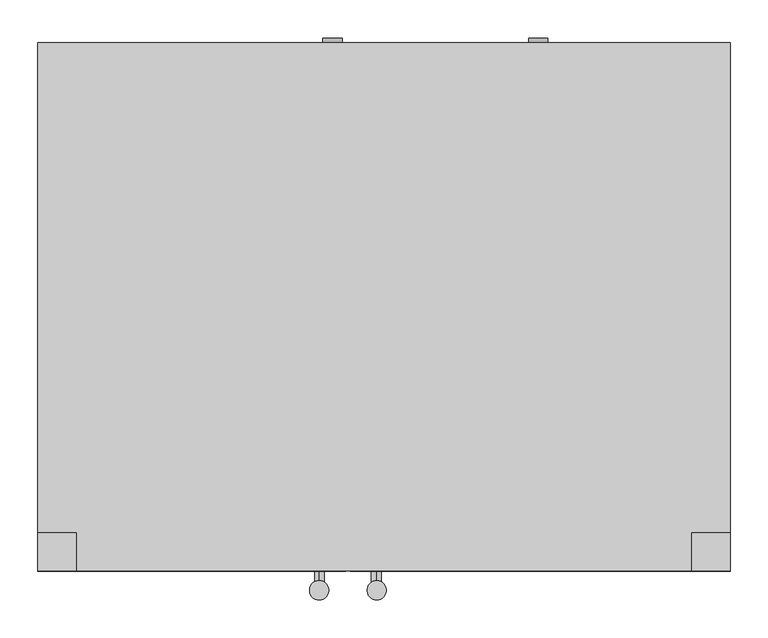
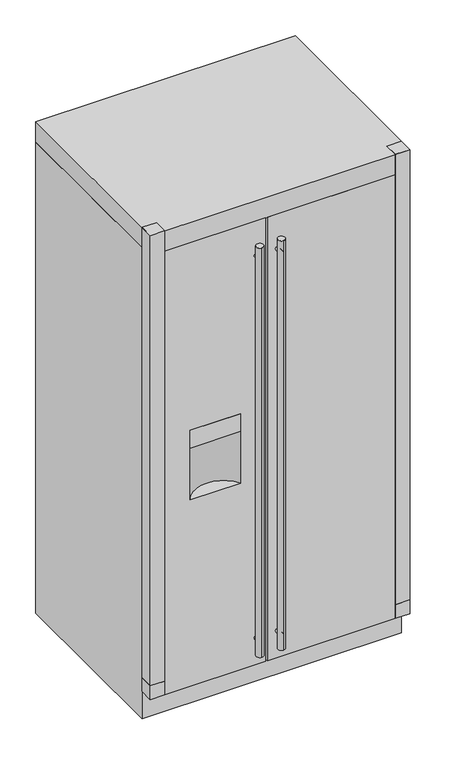
"""IFC4 building model written with IfcOpenShell, lengths in millimetres: proxy geometry, Refrige_Side-By-Side_GE-Monogram_ZFSB23DXSS : Refrige_Side-By-Side_GE-Monogram_ZFSB23DXSS."""

from ifc_helpers import new_model, si_unit, point, frame, frame_2d, origin, origin_with_axes, place, context, project, spatial, polyline, circle_curve, trimmed, segment, composite_curve, outline, extrude, faceted_brep, source, transform, mapped, element, save
from ifc_brep_helpers import plane_surface, revolved_surface, advanced_brep


def specialty_equipment_95538555(model_context):
    return source(origin(), model_context, "Body", "SolidModel", [
        extrude(outline(composite_curve([segment(trimmed(circle_curve(frame_2d((203.2, -10.2065026)), 6.35), [point((196.85, -10.2065026))], [point((209.55, -10.2065026))], False, "CARTESIAN"), True, "CONTINUOUS"), segment(trimmed(circle_curve(frame_2d((203.2, -10.2065026)), 6.35), [point((209.55, -10.2065026))], [point((196.85, -10.2065026))], False, "CARTESIAN"), True, "CONTINUOUS")], self_intersect=False)), frame((0.0, -546.1, 0.0), z_axis=(0.0, 1.0, 0.0), x_axis=(0.0, 0.0, 1.0)), (0.0, 0.0, 1.0), 25.4),
        extrude(outline(composite_curve([segment(trimmed(circle_curve(frame_2d((1625.6, -10.2065026)), 6.35), [point((1619.25, -10.2065026))], [point((1631.95, -10.2065026))], False, "CARTESIAN"), True, "CONTINUOUS"), segment(trimmed(circle_curve(frame_2d((1625.6, -10.2065026)), 6.35), [point((1631.95, -10.2065026))], [point((1619.25, -10.2065026))], False, "CARTESIAN"), True, "CONTINUOUS")], self_intersect=False)), frame((0.0, -546.1, 0.0), z_axis=(0.0, 1.0, 0.0), x_axis=(0.0, 0.0, 1.0)), (0.0, 0.0, 1.0), 25.4),
        extrude(outline(composite_curve([segment(trimmed(circle_curve(frame_2d((-9.7026178, -546.1)), 12.7), [point((-9.7026178, -558.8))], [point((-9.7026178, -533.4))], False, "CARTESIAN"), True, "CONTINUOUS"), segment(trimmed(circle_curve(frame_2d((-9.7026178, -546.1)), 12.7), [point((-9.7026178, -533.4))], [point((-9.7026178, -558.8))], False, "CARTESIAN"), True, "CONTINUOUS")], self_intersect=False)), frame((0.0, 0.0, 152.4), z_axis=(0.0, 0.0, 1.0), x_axis=(1.0, 0.0, 0.0)), (0.0, 0.0, 1.0), 1524.0),
        extrude(outline(composite_curve([segment(trimmed(circle_curve(frame_2d((203.2, -85.1990605)), 6.35), [point((196.85, -85.1990605))], [point((209.55, -85.1990605))], False, "CARTESIAN"), True, "CONTINUOUS"), segment(trimmed(circle_curve(frame_2d((203.2, -85.1990605)), 6.35), [point((209.55, -85.1990605))], [point((196.85, -85.1990605))], False, "CARTESIAN"), True, "CONTINUOUS")], self_intersect=False)), frame((0.0, -546.1, 0.0), z_axis=(0.0, 1.0, 0.0), x_axis=(0.0, 0.0, 1.0)), (0.0, 0.0, 1.0), 25.4),
        extrude(outline(composite_curve([segment(trimmed(circle_curve(frame_2d((1625.6, -85.1990605)), 6.35), [point((1619.25, -85.1990605))], [point((1631.95, -85.1990605))], False, "CARTESIAN"), True, "CONTINUOUS"), segment(trimmed(circle_curve(frame_2d((1625.6, -85.1990605)), 6.35), [point((1631.95, -85.1990605))], [point((1619.25, -85.1990605))], False, "CARTESIAN"), True, "CONTINUOUS")], self_intersect=False)), frame((0.0, -546.1, 0.0), z_axis=(0.0, 1.0, 0.0), x_axis=(0.0, 0.0, 1.0)), (0.0, 0.0, 1.0), 25.4),
        extrude(outline(composite_curve([segment(trimmed(circle_curve(frame_2d((-85.7029453, -546.1)), 12.7), [point((-85.7029453, -558.8))], [point((-85.7029453, -533.4))], False, "CARTESIAN"), True, "CONTINUOUS"), segment(trimmed(circle_curve(frame_2d((-85.7029453, -546.1)), 12.7), [point((-85.7029453, -533.4))], [point((-85.7029453, -558.8))], False, "CARTESIAN"), True, "CONTINUOUS")], self_intersect=False)), frame((0.0, 0.0, 152.4), z_axis=(0.0, 0.0, 1.0), x_axis=(1.0, 0.0, 0.0)), (0.0, 0.0, 1.0), 1524.0),
        extrude(outline(composite_curve([segment(trimmed(circle_curve(frame_2d((-228.6, -573.0875)), 103.1875), [point((-317.5, -520.7))], [point((-139.7, -520.7))], False, "CARTESIAN"), True, "CONTINUOUS"), segment(polyline([(-139.7, -520.7), (-317.5, -520.7)]), True, "CONTINUOUS")], self_intersect=False)), frame((0.0, 0.0, 989.0466464), z_axis=(0.0, 0.0, 1.0), x_axis=(1.0, 0.0, 0.0)), (0.0, 0.0, 1.0), 65.7299795),
        extrude(outline(polyline([(-406.4, -469.9), (-406.4, -520.7), (-457.2, -520.7), (-457.2, -469.9), (-406.4, -469.9)])), frame((0.0, 0.0, 101.6), z_axis=(0.0, 0.0, 1.0), x_axis=(1.0, 0.0, 0.0)), (0.0, 0.0, 1.0), 50.8),
        extrude(outline(polyline([(457.2, -469.9), (457.2, -520.7), (406.4, -520.7), (406.4, -469.9), (457.2, -469.9)])), frame((0.0, 0.0, 101.6), z_axis=(0.0, 0.0, 1.0), x_axis=(1.0, 0.0, 0.0)), (0.0, 0.0, 1.0), 50.8),
        extrude(outline(polyline([(-406.4, -469.9), (-406.4, -520.7), (-457.2, -520.7), (-457.2, -469.9), (-406.4, -469.9)])), frame((0.0, 0.0, 101.6), z_axis=(0.0, 0.0, 1.0), x_axis=(1.0, 0.0, 0.0)), (0.0, 0.0, 1.0), 1727.2),
        extrude(outline(polyline([(406.4, -469.9), (457.2, -469.9), (457.2, -520.7), (406.4, -520.7), (406.4, -469.9)])), frame((0.0, 0.0, 101.6), z_axis=(0.0, 0.0, 1.0), x_axis=(1.0, 0.0, 0.0)), (0.0, 0.0, 1.0), 1727.2),
        advanced_brep(
        [(-50.8, -469.9, 1752.6), (-406.4, -469.9, 1752.6), (-406.4, -520.7, 1752.6), (-50.8, -520.7, 1752.6), (-50.8, -469.9, 101.6), (-50.8, -520.7, 101.6), (-406.4, -520.7, 101.6), (-406.4, -469.9, 101.6), (-317.5, -520.7, 1054.7766259), (-139.7, -520.7, 1054.7766259), (-139.7, -520.7, 796.7567269), (-317.5, -520.7, 796.7567269), (-228.6, -469.9, 1054.7766259), (-228.6, -469.9, 796.7567269)],
        [
            (0, 1),
            (1, 2),
            (2, 3),
            (3, 0),
            (4, 5),
            (5, 6),
            (6, 7),
            (7, 4),
            (0, 4),
            (7, 1),
            (6, 2),
            (5, 3),
            (8, 9),
            (9, 10),
            (10, 11),
            (11, 8),
            (8, 12, circle_curve(frame((-228.6, -573.0875, 1054.7766259), z_axis=(0.0, 0.0, -1.0), x_axis=(1.0, 0.0, 0.0)), 103.1875)),
            (12, 9, circle_curve(frame((-228.6, -573.0875, 1054.7766259), z_axis=(0.0, 0.0, -1.0), x_axis=(1.0, 0.0, 0.0)), 103.1875)),
            (10, 13, circle_curve(frame((-228.6, -573.0875, 796.7567269), z_axis=(0.0, 0.0, 1.0), x_axis=(1.0, 0.0, 0.0)), 103.1875)),
            (13, 11, circle_curve(frame((-228.6, -573.0875, 796.7567269), z_axis=(0.0, 0.0, 1.0), x_axis=(1.0, 0.0, 0.0)), 103.1875)),
        ],
        [
            plane_surface(frame((-406.4, -469.9, 1752.6), z_axis=(0.0, 0.0, 1.0), x_axis=(-1.0, 0.0, 0.0))),
            plane_surface(frame((-406.4, -469.9, 101.6), z_axis=(0.0, 0.0, -1.0), x_axis=(1.0, 0.0, 0.0))),
            plane_surface(frame((-50.8, -469.9, 1752.6), z_axis=(0.0, 1.0, 0.0), x_axis=(0.0, 0.0, -1.0))),
            plane_surface(frame((-406.4, -469.9, 1752.6), z_axis=(-1.0, 0.0, 0.0), x_axis=(0.0, 0.0, -1.0))),
            plane_surface(frame((-406.4, -520.7, 1752.6), z_axis=(0.0, -1.0, 0.0), x_axis=(0.0, 0.0, -1.0))),
            plane_surface(frame((-50.8, -520.7, 1752.6), z_axis=(1.0, 0.0, 0.0), x_axis=(0.0, 0.0, -1.0))),
            plane_surface(frame((-139.7, -520.7, 1054.7766259), z_axis=(0.0, 0.0, -1.0), x_axis=(1.0, 0.0, 0.0))),
            plane_surface(frame((-139.7, -520.7, 796.7567269), z_axis=(0.0, 0.0, 1.0), x_axis=(-1.0, 0.0, 0.0))),
            revolved_surface(polyline([(-125.4125, -573.0875, 1054.7766259), (-125.4125, -573.0875, 796.7567269)]), (-228.6, -573.0875, 796.7567269), (0.0, 0.0, 1.0)),
        ],
        [
            (0, [[1, 2, 3, 4]]),
            (1, [[5, 6, 7, 8]]),
            (2, [[-1, 9, -8, 10]]),
            (3, [[-2, -10, -7, 11]]),
            (4, [[-3, -11, -6, 12], [13, 14, 15, 16]]),
            (5, [[-4, -12, -5, -9]]),
            (6, [[17, 18, -13]]),
            (7, [[19, 20, -15]]),
            (8, [[-17, -16, -20, -19, -14, -18]]),
        ],
    ),
        faceted_brep([(406.4, -469.9, 1752.6), (-44.45, -469.9, 1752.6), (-44.45, -520.7, 1752.6), (406.4, -520.7, 1752.6), (406.4, -469.9, 101.6), (406.4, -520.7, 101.6), (-44.45, -520.7, 101.6), (-44.45, -469.9, 101.6)], [[[0, 1, 2, 3]], [[4, 5, 6, 7]], [[1, 0, 4, 7]], [[2, 1, 7, 6]], [[3, 2, 6, 5]], [[0, 3, 5, 4]]]),
        extrude(outline(polyline([(457.2, -469.9), (-457.2, -469.9), (-457.2, 177.8), (457.2, 177.8), (457.2, -469.9)])), origin_with_axes(), (0.0, 0.0, 1.0), 1752.6),
        extrude(outline(polyline([(-457.2, -520.7), (-457.2, 177.8), (457.2, 177.8), (457.2, -520.7), (-457.2, -520.7)])), frame((0.0, 0.0, 1752.6), z_axis=(0.0, 0.0, 1.0), x_axis=(1.0, 0.0, 0.0)), (0.0, 0.0, 1.0), 76.2),
        extrude(outline(composite_curve([segment(trimmed(circle_curve(frame_2d((314.6288473, -68.0887314)), 12.7), [point((314.6288473, -55.3887314))], [point((314.6288473, -80.7887314))], False, "CARTESIAN"), True, "CONTINUOUS"), segment(trimmed(circle_curve(frame_2d((314.6288473, -68.0887314)), 12.7), [point((314.6288473, -80.7887314))], [point((314.6288473, -55.3887314))], False, "CARTESIAN"), True, "CONTINUOUS")], self_intersect=False)), frame((0.0, 177.8, 0.0), z_axis=(0.0, 1.0, 0.0), x_axis=(0.0, 0.0, 1.0)), (0.0, 0.0, 1.0), 6.35),
        extrude(outline(composite_curve([segment(trimmed(circle_curve(frame_2d((314.6288473, 203.7929589)), 12.7), [point((314.6288473, 216.4929589))], [point((314.6288473, 191.0929589))], False, "CARTESIAN"), True, "CONTINUOUS"), segment(trimmed(circle_curve(frame_2d((314.6288473, 203.7929589)), 12.7), [point((314.6288473, 191.0929589))], [point((314.6288473, 216.4929589))], False, "CARTESIAN"), True, "CONTINUOUS")], self_intersect=False)), frame((0.0, 177.8, 0.0), z_axis=(0.0, 1.0, 0.0), x_axis=(0.0, 0.0, 1.0)), (0.0, 0.0, 1.0), 6.35),
    ])


if __name__ == "__main__":
    model = new_model("IFC4")
    model_context = context("Model", 3, world=origin())
    ifc_project = project(units=[si_unit("LENGTHUNIT", "METRE", prefix="MILLI")], contexts=[model_context])
    site = spatial("IfcSite", under=ifc_project)
    building = spatial("IfcBuilding", under=site)
    placement = place(None, origin())
    specialty_equipment_shape = specialty_equipment_95538555(model_context)
    element("IfcBuildingElementProxy", 1, Name="Refrige_Side-By-Side_GE-Monogram_ZFSB23DXSS : Refrige_Side-By-Side_GE-Monogram_ZFSB23DXSS", ObjectType="Refrige_Side-By-Side_GE-Monogram_ZFSB23DXSS : Refrige_Side-By-Side_GE-Monogram_ZFSB23DXSS", at=placement, inside=building, context=model_context, shape_type="MappedRepresentation", body=[
        mapped(specialty_equipment_shape, transform((0.0, 0.0, 0.0), x_axis=(1.0, 0.0, 0.0), y_axis=(0.0, 1.0, 0.0), z_axis=(0.0, 0.0, 1.0))),
    ])
    save(model, "model.ifc")

# Revit data of these elements
# Type "Refrige_Side-By-Side_GE-Monogram_ZFSB23DXSS : Refrige_Side-By-Side_GE-Monogram_ZFSB23DXSS"
#   COBie.Type.CreatedBy = "design@eagle.com"
#   COBie.Type.CreatedOn = "2016-10-27T05:31:12"
#   COBie.Type.Name = "Refrige_Side-By-Side_GE-Monogram_ZFSB23DXSS_Refrige_Side-By-Side_GE-Monogram_ZFSB23DXSS"
#   COBie.Type.Category = "23-40 40 11 11 17 : Refrigerator-Freezer"
#   COBie.Type.Description = "Refrige_Side-By-Side_GE-Monogram_ZFSB23DXSS_Refrige_Side-By-Side_GE-Monogram_ZFSB23DXSS"
#   COBie.Type.Manufacturer = "info@geappliances.com"
#   COBie.Type.ModelNumber = "As Specified in 11 30 00"
#   URL = "http://www.geappliances.com/"
#   Test Data = "http://www.geappliances.com/service_and_support/search.htm"
#   Specification = "http://www.arcat.com/sdspecs/htm/11450gea.htm"
#   SpecWizard = "http://www.arcat.com/specwizard/11450gea/index.htm?mf=&coid=32703"
#   Send Message = "http://www.arcat.com/users.pl?action=UserEmail&company=GE%20Appliances&coid=32703&rep=114&fax=502-452-0620&mf="
#   Sales Information = "http://www.geappliances.com/buy/"
#   Revision = "R1_02-2011"
#   Product Properties = "http://www.arcat.com/bim/bim_info.pl?fn=GEAppliances"
#   Product Data = "http://www.arcat.com/arcatcos/cos32/arc32703.html"
#   Model = "As Specified in 11 30 00"
#   Manufacturer Website = "http://www.geappliances.com/"
#   Manufacturer Phone - Toll Free = "800-626-2000"
#   Manufacturer Phone = "502-452-3346"
#   Manufacturer Fax = "502-452-0620"
#   Manufacturer Address = "Appliance Park AP4-109, Louisville, KY 40225"
#   Manufacturer = "info@geappliances.com"
#   Keynote = "11 30 00"
#   Installation-Fabrication = "http://www.geappliances.com/service_and_support/literature/"
#   Installation Phase = ""
#   Green Building-LEED = "http://www.geappliances.com/energy-star-appliances/"
#   ENERGYSTAR Qualified = ""
#   Drawn By = "Sumex Design, Inc. / Robert S. Weygant, CSI, CDT, SCIP"
#   Description = "Residential Appliance as Specified in 11 30 00"
#   Copyright = "©Arcat Inc."
#   Construction Details = "http://www.geappliances.com/design_center/"
#   Capacity = ""
#   Building Codes = "http://www.geappliances.com/service_and_support/search.htm"
#   Assembly Code = "E1090400"
#   COBie.Type.ReplacementCost = 0
#   offset [instance default] = 0' - 0"
#   Voltage_MEP = 120 V
#   Unit Width = 3' - 0"
#   Unit Height = 6' - 0"
#   Unit Depth = 2' - 3 1/2"
#   MEP Apparent Power = 60 VA
#   MEP Amperage = 0.5 A
#   Handle Height [instance default] = 5' - 0"
#   HWRad = 0' - 0 1/4"
#   GasRad = 0' - 0 1/4"
#   DrainRad = 0' - 0 5/8"
#   Connection Dia HW = 0' - 0 1/2"
#   Connection Dia Gas = 0' - 0 1/2"
#   Connection Dia DWV = 0' - 1 1/4"
#   Connection Dia CW = 0' - 0 1/2"
#   CWRad = 0' - 0 1/4"
#   COBie.Type = yes
#   Warranty Duration (Years) = 0
#   Maintenance Schedule (Months) = 0
#   Expected Lifespan (Years) = 0
#   ADA Compliant = yes
#   Handle Finish = none
#   Exterior Finish = ARCAT - Finish Stainless Steel
# Element 1 (IfcBuildingElementProxy, "Refrige_Side-By-Side_GE-Monogram_ZFSB23DXSS : Refrige_Side-By-Side_GE-Monogram_ZFSB23DXSS")
#   Materials on its faces: "ARCAT - Finish Stainless Steel", "Cold", "Connector"
# Materials
#   "ARCAT - Finish Stainless Steel": class "Unassigned", colour RGB 247 247 247, transparency 0, Keynote = "05050", Model = "Generic", Manufacturer = "Generic", Description = "Steel, Chrome Plated"
#   "Cold": class "Miscellaneous", colour RGB 0 0 255, transparency 0
#   "Connector": class "Miscellaneous", colour RGB 255 255 0, transparency 0
